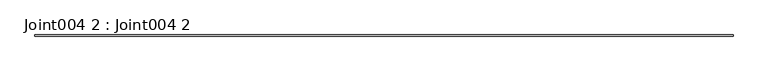
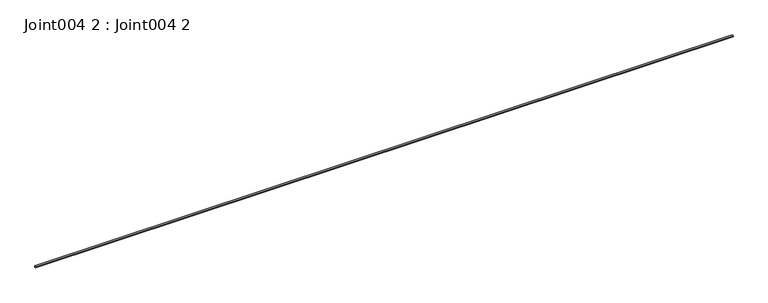
"""IFC4 building model written with IfcOpenShell, lengths in millimetres: proxy geometry, Joint004 2 : Joint004 2."""

from ifc_helpers import new_model, si_unit, point, frame, frame_2d, origin, place, context, project, spatial, polyline, circle_curve, trimmed, segment, composite_curve, outline, extrude, source, transform, mapped, element, save


def joint004_2_joint004_2_8d49f665(model_context):
    return source(origin(), model_context, "Body", "SweptSolid", [
        extrude(outline(composite_curve([segment(polyline([(10405.3793386, 40791.8007813), (10405.3793386, 40795.71875)]), True, "CONTINUOUS"), segment(trimmed(circle_curve(frame_2d((10406.9776706, 40800.890625)), 5.4132205), [point((10405.3793386, 40795.71875))], [point((10408.5760026, 40795.71875))], True, "CARTESIAN"), True, "CONTINUOUS"), segment(polyline([(10408.5760026, 40795.71875), (10408.5760026, 40791.8007813)]), True, "CONTINUOUS"), segment(trimmed(circle_curve(frame_2d((10406.9776706, 40796.9726563)), 5.4132205), [point((10408.5760026, 40791.8007813))], [point((10405.3793386, 40791.8007813))], False, "CARTESIAN"), True, "CONTINUOUS")], self_intersect=False)), frame((3694.2883192, 0.0, 0.0), z_axis=(1.0, 0.0, 0.0), x_axis=(0.0, 1.0, 0.0)), (0.0, 0.0, 1.0), 2000.0),
    ])


if __name__ == "__main__":
    model = new_model("IFC4")
    model_context = context("Model", 3, world=origin())
    ifc_project = project(units=[si_unit("LENGTHUNIT", "METRE", prefix="MILLI")], contexts=[model_context])
    site = spatial("IfcSite", under=ifc_project)
    building = spatial("IfcBuilding", under=site)
    placement = place(None, origin())
    joint004_2_joint004_2_shape = joint004_2_joint004_2_8d49f665(model_context)
    element("IfcBuildingElementProxy", 1, Name="Joint004 2 : Joint004 2", ObjectType="Joint004 2 : Joint004 2", at=placement, inside=building, context=model_context, shape_type="MappedRepresentation", body=[
        mapped(joint004_2_joint004_2_shape, transform((0.0, 0.0, 0.0), x_axis=(1.0, 0.0, 0.0), y_axis=(0.0, 1.0, 0.0), z_axis=(0.0, 0.0, 1.0))),
    ])
    save(model, "model.ifc")

# Revit data of these elements
# Type "Joint004 2 : Joint004 2"
#   NameOverride = "Joint004"
# Element 1 (IfcBuildingElementProxy, "Joint004 2 : Joint004 2")
#   Materials on its faces: "SEALANT JOINT"
# Materials
#   "SEALANT JOINT": class "Unassigned", colour RGB 142 225 148, transparency 0
